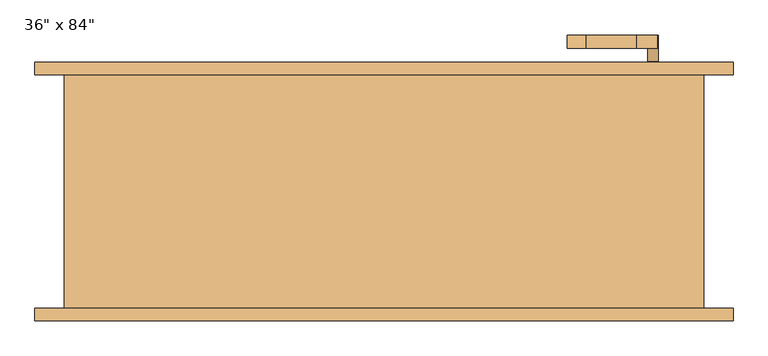
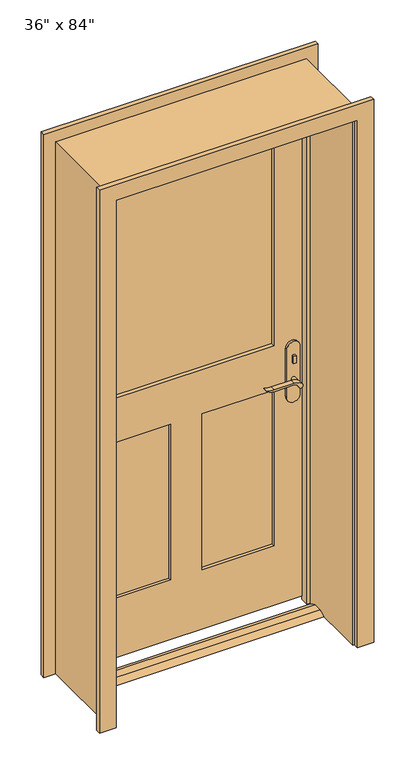
"""IFC4 building model written with IfcOpenShell, lengths in millimetres: door geometry."""

from ifc_helpers import new_model, si_unit, point, frame, frame_2d, origin, place, context, project, spatial, polyline, circle_curve, trimmed, segment, composite_curve, outline, extrude, faceted_brep, source, transform, mapped, element, save


def door_b73f7f09(model_context):
    return source(origin(), model_context, "Body", "SolidModel", [
        extrude(outline(polyline([(38.1, 12.7), (73.025, 12.7), (98.425, 0.0), (12.7, 0.0), (38.1, 12.7)])), frame((-457.2, 0.0, 0.0), z_axis=(1.0, 0.0, 0.0), x_axis=(0.0, 1.0, 0.0)), (0.0, 0.0, 1.0), 914.4),
        extrude(outline(polyline([(411.4, 118.1125), (401.4, 118.1125), (401.4, 128.1125), (411.4, 128.1125), (411.4, 118.1125)])), frame((0.0, 0.0, 981.9), z_axis=(0.0, 0.0, 1.0), x_axis=(1.0, 0.0, 0.0)), (0.0, 0.0, 1.0), 30.0),
        extrude(outline(composite_curve([segment(trimmed(circle_curve(frame_2d((996.9, 406.4)), 8.0), [point((996.9, 398.4))], [point((996.9, 414.4))], False, "CARTESIAN"), True, "CONTINUOUS"), segment(trimmed(circle_curve(frame_2d((996.9, 406.4)), 8.0), [point((996.9, 414.4))], [point((996.9, 398.4))], False, "CARTESIAN"), True, "CONTINUOUS")], self_intersect=False)), frame((0.0, 183.0375, 0.0), z_axis=(0.0, 1.0, 0.0), x_axis=(0.0, 0.0, 1.0)), (0.0, 0.0, 1.0), 10.0),
        extrude(outline(composite_curve([segment(trimmed(circle_curve(frame_2d((897.1555521, 382.7324871)), 37.2832219), [point((919.0523287, 412.9081363))], [point((934.4, 381.0325667))], False, "CARTESIAN"), True, "CONTINUOUS"), segment(polyline([(934.4, 381.0325667), (934.4, 304.7564091)]), True, "CONTINUOUS"), segment(trimmed(circle_curve(frame_2d((1017.6850638, 304.8227909)), 83.2850902), [point((934.4, 304.7564091))], [point((939.4, 276.4))], True, "CARTESIAN"), True, "CONTINUOUS"), segment(polyline([(939.4, 276.4), (936.6135558, 276.4)]), True, "CONTINUOUS"), segment(trimmed(circle_curve(frame_2d((986.6709207, 308.3396612)), 59.3791355), [point((936.6135558, 276.4))], [point((927.4, 304.7564091))], False, "CARTESIAN"), True, "CONTINUOUS"), segment(polyline([(927.4, 304.7564091), (927.4, 381.0138099)]), True, "CONTINUOUS"), segment(trimmed(circle_curve(frame_2d((909.2738613, 381.0138099)), 18.1261387), [point((927.4, 381.0138099))], [point((914.4, 398.4))], True, "CARTESIAN"), True, "CONTINUOUS"), segment(trimmed(circle_curve(frame_2d((914.4, 406.4)), 8.0), [point((914.4, 398.4))], [point((919.0523287, 412.9081363))], False, "CARTESIAN"), True, "CONTINUOUS")], self_intersect=False)), frame((0.0, 78.1125, 0.0), z_axis=(0.0, 1.0, 0.0), x_axis=(0.0, 0.0, 1.0)), (0.0, 0.0, 1.0), 20.0),
        extrude(outline(composite_curve([segment(trimmed(circle_curve(frame_2d((914.4, 406.4)), 8.0), [point((914.3999903, 398.4))], [point((919.0523287, 412.9081363))], False, "CARTESIAN"), True, "CONTINUOUS"), segment(trimmed(circle_curve(frame_2d((897.1555521, 382.7324871)), 37.2832219), [point((919.0523287, 412.9081363))], [point((934.4, 381.0325667))], False, "CARTESIAN"), True, "CONTINUOUS"), segment(polyline([(934.4, 381.0325667), (934.4, 304.7564091)]), True, "CONTINUOUS"), segment(trimmed(circle_curve(frame_2d((1017.6850638, 304.8227909)), 83.2850902), [point((934.4, 304.7564091))], [point((939.4, 276.4))], True, "CARTESIAN"), True, "CONTINUOUS"), segment(polyline([(939.4, 276.4), (936.6135558, 276.4)]), True, "CONTINUOUS"), segment(trimmed(circle_curve(frame_2d((986.6709207, 308.3396612)), 59.3791355), [point((936.6135558, 276.4))], [point((927.4, 304.7564091))], False, "CARTESIAN"), True, "CONTINUOUS"), segment(polyline([(927.4, 304.7564091), (927.4, 381.0138122)]), True, "CONTINUOUS"), segment(trimmed(circle_curve(frame_2d((909.2738682, 381.0138122)), 18.1261318), [point((927.4, 381.0138122))], [point((914.3999903, 398.4))], True, "CARTESIAN"), True, "CONTINUOUS")], self_intersect=False)), frame((0.0, 213.0375, 0.0), z_axis=(0.0, 1.0, 0.0), x_axis=(0.0, 0.0, 1.0)), (0.0, 0.0, 1.0), 20.0),
        extrude(outline(composite_curve([segment(trimmed(circle_curve(frame_2d((914.4, 406.4)), 8.0), [point((914.4, 398.4))], [point((914.4, 414.4))], False, "CARTESIAN"), True, "CONTINUOUS"), segment(trimmed(circle_curve(frame_2d((914.4, 406.4)), 8.0), [point((914.4, 414.4))], [point((914.4, 398.4))], False, "CARTESIAN"), True, "CONTINUOUS")], self_intersect=False)), frame((0.0, 98.1125, 0.0), z_axis=(0.0, 1.0, 0.0), x_axis=(0.0, 0.0, 1.0)), (0.0, 0.0, 1.0), 30.0),
        extrude(outline(composite_curve([segment(trimmed(circle_curve(frame_2d((914.4, 406.4)), 8.0), [point((914.4, 398.4))], [point((914.4, 414.4))], False, "CARTESIAN"), True, "CONTINUOUS"), segment(trimmed(circle_curve(frame_2d((914.4, 406.4)), 8.0), [point((914.4, 414.4))], [point((914.4, 398.4))], False, "CARTESIAN"), True, "CONTINUOUS")], self_intersect=False)), frame((0.0, 183.0375, 0.0), z_axis=(0.0, 1.0, 0.0), x_axis=(0.0, 0.0, 1.0)), (0.0, 0.0, 1.0), 30.0),
        extrude(outline(composite_curve([segment(polyline([(844.4, 431.4), (1039.4, 431.4)]), True, "CONTINUOUS"), segment(trimmed(circle_curve(frame_2d((1039.4, 406.4)), 25.0), [point((1039.4, 431.4))], [point((1039.4, 381.4))], False, "CARTESIAN"), True, "CONTINUOUS"), segment(polyline([(1039.4, 381.4), (844.4, 381.4)]), True, "CONTINUOUS"), segment(trimmed(circle_curve(frame_2d((844.4, 406.4)), 25.0), [point((844.4, 381.4))], [point((844.4, 431.4))], False, "CARTESIAN"), True, "CONTINUOUS")], self_intersect=False)), frame((0.0, 128.1125, 0.0), z_axis=(0.0, 1.0, 0.0), x_axis=(0.0, 0.0, 1.0)), (0.0, 0.0, 1.0), 10.0),
        extrude(outline(composite_curve([segment(polyline([(844.4, 431.4), (1039.4, 431.4)]), True, "CONTINUOUS"), segment(trimmed(circle_curve(frame_2d((1039.4, 406.4)), 25.0), [point((1039.4, 431.4))], [point((1039.4, 381.4))], False, "CARTESIAN"), True, "CONTINUOUS"), segment(polyline([(1039.4, 381.4), (844.4, 381.4)]), True, "CONTINUOUS"), segment(trimmed(circle_curve(frame_2d((844.4, 406.4)), 25.0), [point((844.4, 381.4))], [point((844.4, 431.4))], False, "CARTESIAN"), True, "CONTINUOUS")], self_intersect=False)), frame((0.0, 173.0375, 0.0), z_axis=(0.0, 1.0, 0.0), x_axis=(0.0, 0.0, 1.0)), (0.0, 0.0, 1.0), 10.0),
        extrude(outline(polyline([(2133.6, -457.2), (12.7, -457.2), (12.7, 457.2), (2133.6, 457.2), (2133.6, -457.2)]), holes=[polyline([(1066.8, -336.55), (2012.95, -336.55), (2012.95, 336.55), (1066.8, 336.55), (1066.8, -336.55)]), polyline([(885.825, -60.325), (254.0, -60.325), (254.0, -336.55), (885.825, -336.55), (885.825, -60.325)]), polyline([(885.825, 336.55), (254.0, 336.55), (254.0, 60.325), (885.825, 60.325), (885.825, 336.55)])]), frame((0.0, 138.1125, 0.0), z_axis=(0.0, 1.0, 0.0), x_axis=(0.0, 0.0, 1.0)), (0.0, 0.0, 1.0), 34.925),
        faceted_brep([(482.6, 173.0375, 0.0), (482.6, -179.3875, 0.0), (457.2, -179.3875, 0.0), (457.2, 103.1875, 0.0), (444.5, 103.1875, 0.0), (444.5, 138.1125, 0.0), (457.2, 138.1125, 0.0), (457.2, 173.0375, 0.0), (482.6, 173.0375, 2159.0), (482.6, -179.3875, 2159.0), (-482.6, -179.3875, 2159.0), (-482.6, -179.3875, 0.0), (-457.2, -179.3875, 0.0), (-457.2, -179.3875, 2133.6), (457.2, -179.3875, 2133.6), (457.2, 103.1875, 2133.6), (-457.2, 103.1875, 2133.6), (-457.2, 103.1875, 0.0), (-444.5, 103.1875, 0.0), (-444.5, 103.1875, 2120.9), (444.5, 103.1875, 2120.9), (444.5, 138.1125, 2120.9), (-444.5, 138.1125, 2120.9), (-444.5, 138.1125, 0.0), (-457.2, 138.1125, 0.0), (-457.2, 138.1125, 2133.6), (457.2, 138.1125, 2133.6), (457.2, 173.0375, 2133.6), (-457.2, 173.0375, 2133.6), (-457.2, 173.0375, 0.0), (-482.6, 173.0375, 0.0), (-482.6, 173.0375, 2159.0)], [[[0, 1, 2, 3, 4, 5, 6, 7]], [[1, 0, 8, 9]], [[2, 1, 9, 10, 11, 12, 13, 14]], [[3, 2, 14, 15]], [[4, 3, 15, 16, 17, 18, 19, 20]], [[5, 4, 20, 21]], [[6, 5, 21, 22, 23, 24, 25, 26]], [[7, 6, 26, 27]], [[0, 7, 27, 28, 29, 30, 31, 8]], [[9, 8, 31, 10]], [[15, 14, 13, 16]], [[21, 20, 19, 22]], [[27, 26, 25, 28]], [[30, 29, 24, 23, 18, 17, 12, 11]], [[10, 31, 30, 11]], [[16, 13, 12, 17]], [[22, 19, 18, 23]], [[28, 25, 24, 29]]]),
        extrude(outline(polyline([(-60.325, 149.7541667), (-336.55, 149.7541667), (-336.55, 161.3958333), (-60.325, 161.3958333), (-60.325, 149.7541667)])), frame((0.0, 0.0, 254.0), z_axis=(0.0, 0.0, 1.0), x_axis=(1.0, 0.0, 0.0)), (0.0, 0.0, 1.0), 631.825),
        extrude(outline(polyline([(336.55, 149.7541667), (60.325, 149.7541667), (60.325, 161.3958333), (336.55, 161.3958333), (336.55, 149.7541667)])), frame((0.0, 0.0, 254.0), z_axis=(0.0, 0.0, 1.0), x_axis=(1.0, 0.0, 0.0)), (0.0, 0.0, 1.0), 631.825),
        extrude(outline(polyline([(336.55, 152.0825), (-336.55, 152.0825), (-336.55, 159.0675), (336.55, 159.0675), (336.55, 152.0825)])), frame((0.0, 0.0, 1066.8), z_axis=(0.0, 0.0, 1.0), x_axis=(1.0, 0.0, 0.0)), (0.0, 0.0, 1.0), 946.15),
        extrude(outline(polyline([(0.0, -527.05), (0.0, -463.55), (2139.95, -463.55), (2139.95, 463.55), (0.0, 463.55), (0.0, 527.05), (2203.45, 527.05), (2203.45, -527.05), (0.0, -527.05)])), frame((0.0, -198.4375, 0.0), z_axis=(0.0, 1.0, 0.0), x_axis=(0.0, 0.0, 1.0)), (0.0, 0.0, 1.0), 19.05),
        extrude(outline(polyline([(0.0, -527.05), (0.0, -463.55), (2139.95, -463.55), (2139.95, 463.55), (0.0, 463.55), (0.0, 527.05), (2203.45, 527.05), (2203.45, -527.05), (0.0, -527.05)])), frame((0.0, 173.0375, 0.0), z_axis=(0.0, 1.0, 0.0), x_axis=(0.0, 0.0, 1.0)), (0.0, 0.0, 1.0), 19.05),
    ])


if __name__ == "__main__":
    model = new_model("IFC4")
    model_context = context("Model", 3, world=origin())
    ifc_project = project(units=[si_unit("LENGTHUNIT", "METRE", prefix="MILLI")], contexts=[model_context])
    site = spatial("IfcSite", under=ifc_project)
    building = spatial("IfcBuilding", under=site)
    placement = place(None, origin())
    door_shape = door_b73f7f09(model_context)
    element("IfcDoor", 1, ObjectType="Door-Exterior-Single-Entry-Half Flat Glass-Wood_Clad : 36\" x 84\"", at=placement, inside=building, context=model_context, shape_type="MappedRepresentation", body=[
        mapped(door_shape, transform((0.0, 0.0, 0.0), x_axis=(1.0, 0.0, 0.0), y_axis=(0.0, 1.0, 0.0), z_axis=(0.0, 0.0, 1.0))),
    ])
    save(model, "model.ifc")

# Revit data of these elements
# Type "Door-Exterior-Single-Entry-Half Flat Glass-Wood_Clad : 36\" x 84\""
#   Type Mark = "25"
#   Assembly Code = "B2030100"
#   Analytic Construction = "French door, wood frame with single glass"
#   Top Rail = 0' - 4 3/4"
#   Threshold Offset [instance default] = 0' - 0 1/2"
#   Thickness = 0' - 1 3/8"
#   Thermal Resistance (R) = 1.0696 (h·ft²·°F)/BTU
#   Swing Angle [instance default] = 90.0000°
#   Stiles = 0' - 4 3/4"
#   Rough Width = 3' - 2"
#   Rough Height = 7' - 1"
#   Lock Rail = 0' - 7 1/8"
#   Height = 7' - 0"
#   Width = 3' - 0"
#   Heat Transfer Coefficient (U) = 0.9350 BTU/(h·ft²·°F)
#   Door Offset [instance default] = 0' - 0"
#   Bottom Rail = 0' - 9 1/2"
#   Threshold [instance default] = yes
#   Function = 1
#   Exterior Trim [instance default] = yes
#   Trim Material = Cherry
#   Threshold Material = Cherry
#   Panel Material = Cherry
#   Glazing = Glass
#   Frame Material = Cherry
#   Door Handle Material = Aluminum
#   Visual Light Transmittance = 0
#   Solar Heat Gain Coefficient = 0
#   Wall Closure = (empty or 0)
#   Construction Type = (empty or 0)
# Element 1 (IfcDoor, "Door-Exterior-Single-Entry-Half Flat Glass-Wood_Clad : 36\" x 84\"")
#   Materials on its faces: "Cherry", "Aluminum", "Glass"
# Materials
#   "Cherry": class "Wood", colour RGB 226 177 128, transparency 0, Description = "Prunus Serotina", Cost = 0
#   "Glass": class "Glass", colour RGB 0 128 192, transparency 0.75, Description = "Soda Lime Glass", Cost = 0
#   "Aluminum": class "Metal", colour RGB 247 247 247, transparency 0, Description = "Aluminum 6061", Cost = 0
